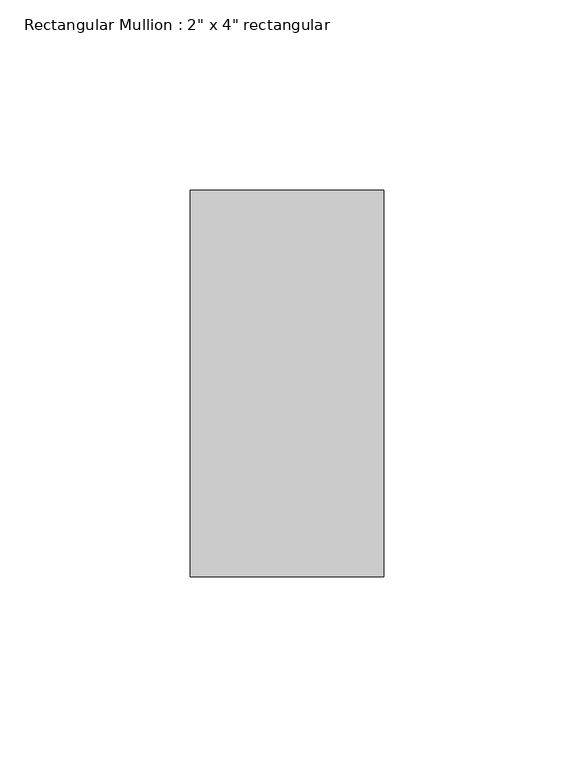
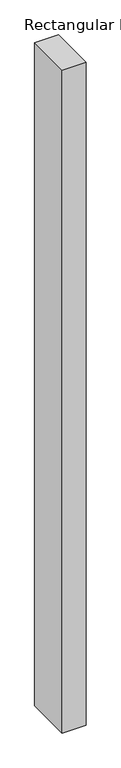
"""IFC4 building model written with IfcOpenShell, lengths in millimetres: member geometry."""

from ifc_helpers import new_model, si_unit, frame, origin, place, context, project, spatial, polyline, outline, extrude, source, transform, mapped, element, save


def member_163854cb(model_context):
    return source(origin(), model_context, "Body", "SweptSolid", [
        extrude(outline(polyline([(0.0, 50.8), (0.0, -50.8), (-50.8, -50.8), (-50.8, 50.8), (0.0, 50.8)])), frame((0.0, 0.0, -1493.1571427), z_axis=(0.0, 0.0, 1.0), x_axis=(1.0, 0.0, 0.0)), (0.0, 0.0, 1.0), 1493.1571427),
    ])


if __name__ == "__main__":
    model = new_model("IFC4")
    model_context = context("Model", 3, world=origin())
    ifc_project = project(units=[si_unit("LENGTHUNIT", "METRE", prefix="MILLI")], contexts=[model_context])
    site = spatial("IfcSite", under=ifc_project)
    building = spatial("IfcBuilding", under=site)
    placement = place(None, origin())
    member_shape = member_163854cb(model_context)
    element("IfcMember", 1, ObjectType="Rectangular Mullion : 2\" x 4\" rectangular", at=placement, inside=building, context=model_context, shape_type="MappedRepresentation", body=[
        mapped(member_shape, transform((0.0, 0.0, 0.0), x_axis=(1.0, 0.0, 0.0), y_axis=(0.0, 1.0, 0.0), z_axis=(0.0, 0.0, 1.0))),
    ])
    save(model, "model.ifc")

# Revit data of these elements
# Type "Rectangular Mullion : 2\" x 4\" rectangular"
#   built-in parameter 1007304 = 0.333333 (stored number, unit not read)
#   built-in parameter 1007301 = 0.0833333 (stored number, unit not read)
#   built-in parameter 1007300 = 0.0833333 (stored number, unit not read)
